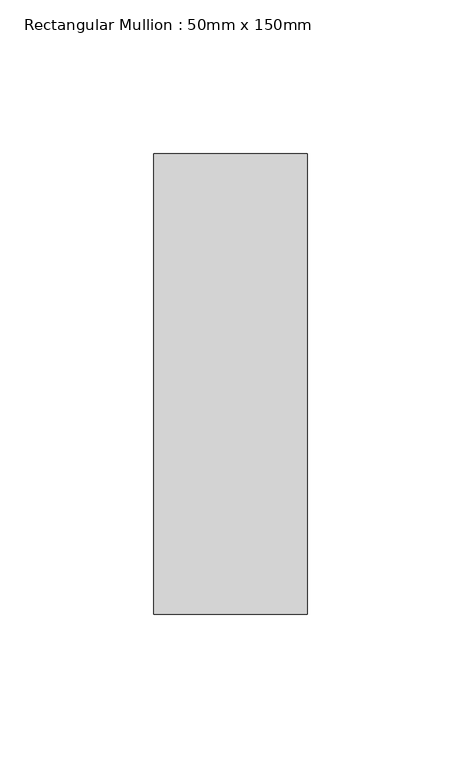
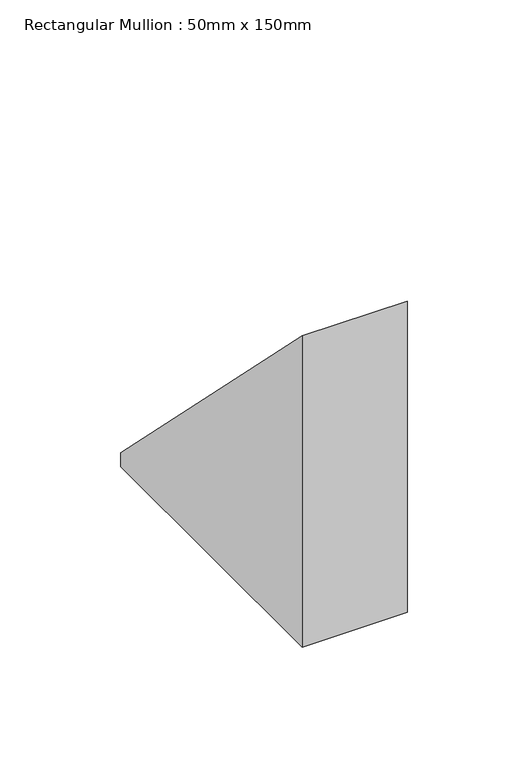
"""IFC4 building model written with IfcOpenShell, lengths in millimetres: member geometry, Rectangular Mullion : 50mm x 150mm."""

from ifc_helpers import new_model, si_unit, frame, origin, place, context, project, spatial, polyline, outline, extrude, source, transform, mapped, element, save


def rectangular_mullion_50mm_x_150mm_894d925c(model_context):
    return source(origin(), model_context, "Body", "SweptSolid", [
        extrude(outline(polyline([(-75.0, 75.0), (75.0, -75.0), (75.0, -82.0909088), (-75.0, -82.0909088), (-75.0, 75.0)])), frame((-25.0, 0.0, 0.0), z_axis=(1.0, 0.0, 0.0), x_axis=(0.0, 1.0, 0.0)), (0.0, 0.0, 1.0), 50.0),
    ])


if __name__ == "__main__":
    model = new_model("IFC4")
    model_context = context("Model", 3, world=origin())
    ifc_project = project(units=[si_unit("LENGTHUNIT", "METRE", prefix="MILLI")], contexts=[model_context])
    site = spatial("IfcSite", under=ifc_project)
    building = spatial("IfcBuilding", under=site)
    placement = place(None, origin())
    rectangular_mullion_50mm_x_150mm_shape = rectangular_mullion_50mm_x_150mm_894d925c(model_context)
    element("IfcMember", 1, ObjectType="Rectangular Mullion : 50mm x 150mm", at=placement, inside=building, context=model_context, shape_type="MappedRepresentation", body=[
        mapped(rectangular_mullion_50mm_x_150mm_shape, transform((0.0, 0.0, 0.0), x_axis=(1.0, 0.0, 0.0), y_axis=(0.0, 1.0, 0.0), z_axis=(0.0, 0.0, 1.0))),
    ])
    save(model, "model.ifc")

# Revit data of these elements
# Type "Rectangular Mullion : 50mm x 150mm"
#   built-in parameter 1007304 = 0.492126 (stored number, unit not read)
#   built-in parameter 1007301 = 0.082021 (stored number, unit not read)
#   built-in parameter 1007300 = 0.082021 (stored number, unit not read)
# Element 1 (IfcMember, "Rectangular Mullion : 50mm x 150mm")
#   Materials on its faces: "Aluminum"
# Materials
#   "Aluminum": class "Metal", colour RGB 244 244 244, transparency 0, Description = "Aluminum 6061", Cost = 0
